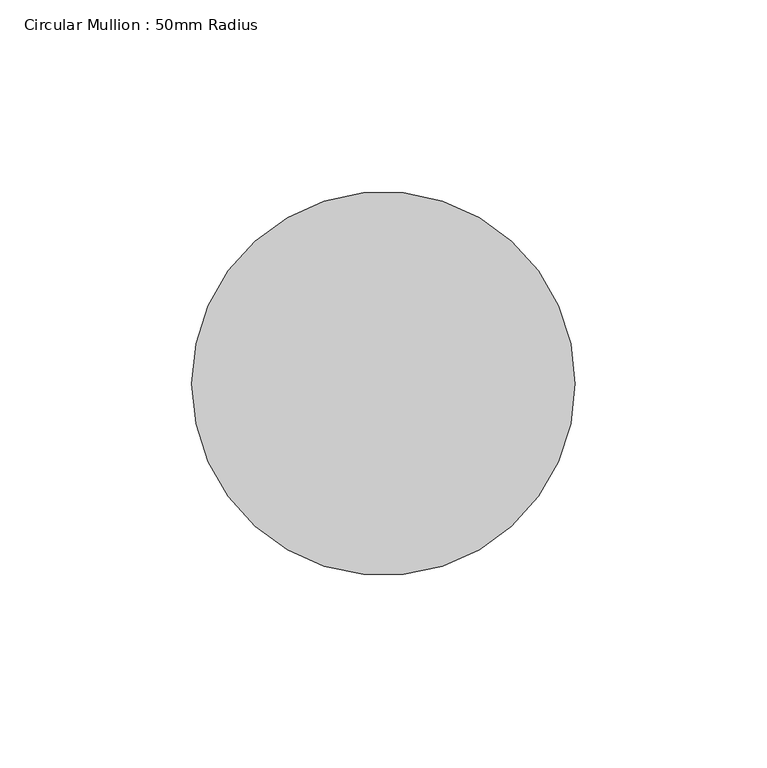
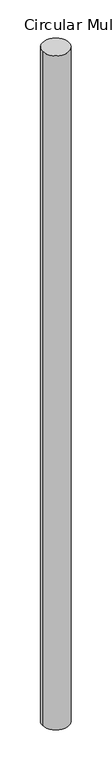
"""IFC4 building model written with IfcOpenShell, lengths in millimetres: member geometry, Circular Mullion : 50mm Radius."""

from ifc_helpers import new_model, si_unit, point, frame, frame_2d, origin, place, context, project, spatial, circle_curve, trimmed, segment, composite_curve, outline, extrude, source, transform, mapped, element, save


def circular_mullion_50mm_radius_f17d88c6(model_context):
    return source(origin(), model_context, "Body", "SweptSolid", [
        extrude(outline(composite_curve([segment(trimmed(circle_curve(frame_2d((-50.0, 0.0)), 50.0), [point((0.0, 0.0))], [point((-100.0, 0.0))], False, "CARTESIAN"), True, "CONTINUOUS"), segment(trimmed(circle_curve(frame_2d((-50.0, 0.0)), 50.0), [point((-100.0, 0.0))], [point((0.0, 0.0))], False, "CARTESIAN"), True, "CONTINUOUS")], self_intersect=False)), frame((0.0, 0.0, -2658.5082898), z_axis=(0.0, 0.0, 1.0), x_axis=(1.0, 0.0, 0.0)), (0.0, 0.0, 1.0), 2658.5082898),
    ])


if __name__ == "__main__":
    model = new_model("IFC4")
    model_context = context("Model", 3, world=origin())
    ifc_project = project(units=[si_unit("LENGTHUNIT", "METRE", prefix="MILLI")], contexts=[model_context])
    site = spatial("IfcSite", under=ifc_project)
    building = spatial("IfcBuilding", under=site)
    placement = place(None, origin())
    circular_mullion_50mm_radius_shape = circular_mullion_50mm_radius_f17d88c6(model_context)
    element("IfcMember", 1, ObjectType="Circular Mullion : 50mm Radius", at=placement, inside=building, context=model_context, shape_type="MappedRepresentation", body=[
        mapped(circular_mullion_50mm_radius_shape, transform((0.0, 0.0, 0.0), x_axis=(1.0, 0.0, 0.0), y_axis=(0.0, 1.0, 0.0), z_axis=(0.0, 0.0, 1.0))),
    ])
    save(model, "model.ifc")

# Revit data of these elements
# Type "Circular Mullion : 50mm Radius"
#   built-in parameter 1007350 = 0.164042 (stored number, unit not read)
# Element 1 (IfcMember, "Circular Mullion : 50mm Radius")
#   Materials on its faces: "Aluminium"
# Materials
#   "Aluminium": class "Metal", colour RGB 247 247 247, transparency 0, Description = "Aluminium 6061", Cost = 0
